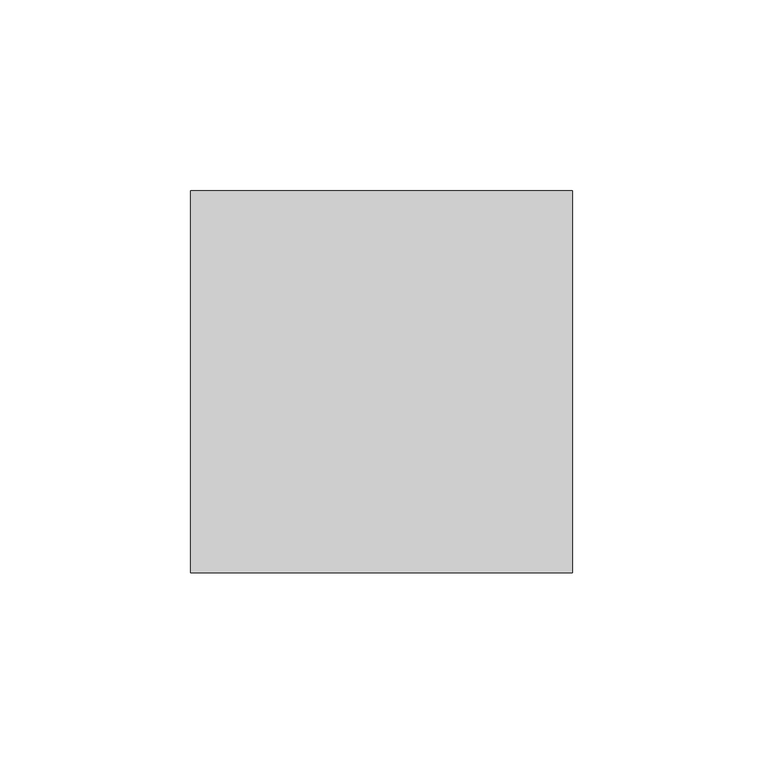
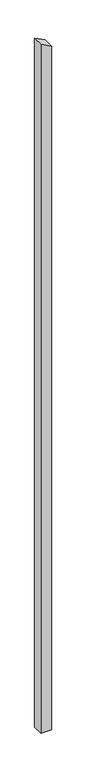
"""IFC4 building model written with IfcOpenShell, lengths in millimetres: column geometry, Holzstütze 159356 : Holzstütze 159356."""

from ifc_helpers import new_model, si_unit, frame, origin, place, context, project, spatial, polyline, outline, extrude, source, transform, mapped, element, save


def column_b2a6b517(model_context):
    return source(origin(), model_context, "Body", "SweptSolid", [
        extrude(outline(polyline([(-500.0, 174197.7593015), (-500.0, 174297.7593015), (6345.7118258, 174297.7593015), (6396.6643707, 174197.7593015), (-500.0, 174197.7593015)])), frame((0.0, 41761.7297978, 0.0), z_axis=(0.0, 1.0, 0.0), x_axis=(0.0, 0.0, 1.0)), (0.0, 0.0, 1.0), 100.0),
    ])


if __name__ == "__main__":
    model = new_model("IFC4")
    model_context = context("Model", 3, world=origin())
    ifc_project = project(units=[si_unit("LENGTHUNIT", "METRE", prefix="MILLI")], contexts=[model_context])
    site = spatial("IfcSite", under=ifc_project)
    building = spatial("IfcBuilding", under=site)
    placement = place(None, origin())
    column_shape = column_b2a6b517(model_context)
    element("IfcColumn", 1, ObjectType="Holzstütze 159356 : Holzstütze 159356", at=placement, inside=building, context=model_context, shape_type="MappedRepresentation", body=[
        mapped(column_shape, transform((0.0, 0.0, 0.0), x_axis=(1.0, 0.0, 0.0), y_axis=(0.0, 1.0, 0.0), z_axis=(0.0, 0.0, 1.0))),
    ])
    save(model, "model.ifc")

# Revit data of these elements
# Type "Holzstütze 159356 : Holzstütze 159356"
#   Abrechnungsart = "m"
#   Allright_Bauteil_ID = "0152St 0000143362"
#   Bezeichnung = "Holzstütze"
#   Codetext = "ST-HOLZ\\"
#   Gewerk = "Zimmer- und Holzbauarbeiten"
#   Material = "Holz"
#   Objektname = "Stütze"
#   NameOverride = "Holzstütze"
#   Reference = "Holzstütze"
#   Status = "NEW"
#   ThermalTransmittance = 0.0000 BTU/(h·ft²·°F)
#   Roll = 0.00°
#   Slope = 0.00°
#   2D Interaktion = yes
#   IsExternal = yes
#   LoadBearing = yes
# Element 1 (IfcColumn, "Holzstütze 159356 : Holzstütze 159356")
#   Materials on its faces: "holzschalung"
# Materials
#   "holzschalung": class "Unassigned", colour RGB 128 128 128, transparency 0
